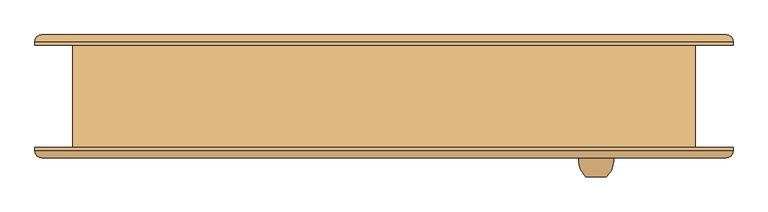
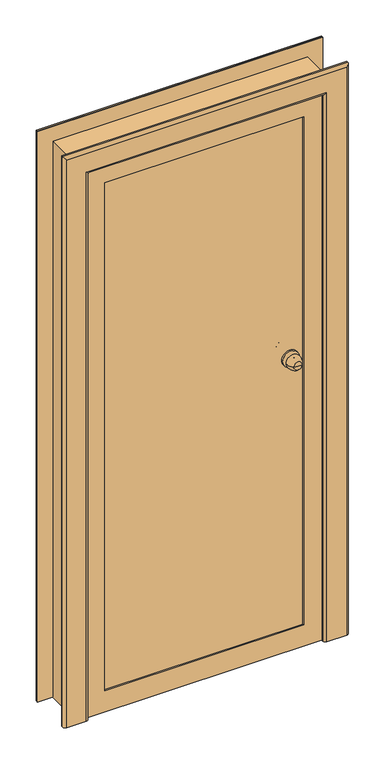
"""IFC4 building model written with IfcOpenShell, lengths in millimetres: door geometry, Наружная дверь 1-Навесная - Один проем наружу с порогом - 31173-2003 : ДСН КЛН  М1 УЗ 2100-910 ГОСТ 31173-2003."""

from ifc_helpers import new_model, si_unit, point, frame, origin, place, context, project, spatial, polyline, circle_curve, ellipse_curve, trimmed, outline, extrude, faceted_brep, source, transform, mapped, element, save
from ifc_brep_helpers import plane_surface, cylinder_surface, revolved_surface, advanced_brep


def door_a4fe4bf0(model_context):
    return source(origin(), model_context, "Body", "SolidModel", [
        advanced_brep(
        [(295.0, -118.0, 1100.0), (310.0, -118.0, 1100.0), (325.0, -118.0, 1100.0), (335.0, -88.0, 1100.0), (285.0, -88.0, 1100.0), (328.0, -88.0, 1100.0), (292.0, -88.0, 1100.0), (320.0, -80.0, 1100.0), (300.0, -80.0, 1100.0), (320.0, -74.0, 1100.0), (300.0, -74.0, 1100.0), (340.0, -74.0, 1100.0), (280.0, -74.0, 1100.0), (340.0, -68.0, 1100.0), (280.0, -68.0, 1100.0)],
        [
            (0, 1),
            (1, 2),
            (2, 0, circle_curve(frame((310.0, -118.0, 1100.0), z_axis=(0.0, -1.0, 0.0), x_axis=(1.0, 0.0, 0.0)), 15.0)),
            (0, 2, circle_curve(frame((310.0, -118.0, 1100.0), z_axis=(0.0, -1.0, 0.0), x_axis=(1.0, 0.0, 0.0)), 15.0)),
            (2, 3, circle_curve(frame((300.3773735, -93.1257912, 1100.0), z_axis=(0.0, 0.0, 1.0), x_axis=(-1.0, 0.0, 0.0)), 35.0)),
            (3, 4, circle_curve(frame((310.0, -88.0, 1100.0), z_axis=(0.0, -1.0, 0.0), x_axis=(1.0, 0.0, 0.0)), 25.0)),
            (4, 0, circle_curve(frame((319.6226265, -93.1257912, 1100.0), z_axis=(0.0, 0.0, 1.0), x_axis=(1.0, 0.0, 0.0)), 35.0)),
            (4, 3, circle_curve(frame((310.0, -88.0, 1100.0), z_axis=(0.0, -1.0, 0.0), x_axis=(1.0, 0.0, 0.0)), 25.0)),
            (3, 5),
            (5, 6, circle_curve(frame((310.0, -88.0, 1100.0), z_axis=(0.0, -1.0, 0.0), x_axis=(1.0, 0.0, 0.0)), 18.0)),
            (6, 4),
            (6, 5, circle_curve(frame((310.0, -88.0, 1100.0), z_axis=(0.0, -1.0, 0.0), x_axis=(1.0, 0.0, 0.0)), 18.0)),
            (5, 7, circle_curve(frame((328.0, -80.0, 1100.0), z_axis=(0.0, 0.0, -1.0), x_axis=(-1.0, 0.0, 0.0)), 8.0)),
            (7, 8, circle_curve(frame((310.0, -80.0, 1100.0), z_axis=(0.0, -1.0, 0.0), x_axis=(1.0, 0.0, 0.0)), 10.0)),
            (8, 6, circle_curve(frame((292.0, -80.0, 1100.0), z_axis=(0.0, 0.0, -1.0), x_axis=(1.0, 0.0, 0.0)), 8.0)),
            (8, 7, circle_curve(frame((310.0, -80.0, 1100.0), z_axis=(0.0, -1.0, 0.0), x_axis=(1.0, 0.0, 0.0)), 10.0)),
            (7, 9),
            (9, 10, circle_curve(frame((310.0, -74.0, 1100.0), z_axis=(0.0, -1.0, 0.0), x_axis=(1.0, 0.0, 0.0)), 10.0)),
            (10, 8),
            (10, 9, circle_curve(frame((310.0, -74.0, 1100.0), z_axis=(0.0, -1.0, 0.0), x_axis=(1.0, 0.0, 0.0)), 10.0)),
            (11, 12, circle_curve(frame((310.0, -74.0, 1100.0), z_axis=(0.0, -1.0, 0.0), x_axis=(-1.0, 0.0, 0.0)), 30.0)),
            (12, 11, circle_curve(frame((310.0, -74.0, 1100.0), z_axis=(0.0, -1.0, 0.0), x_axis=(-1.0, 0.0, 0.0)), 30.0)),
            (13, 14, circle_curve(frame((310.0, -68.0, 1100.0), z_axis=(0.0, 1.0, 0.0), x_axis=(-1.0, 0.0, 0.0)), 30.0)),
            (14, 13, circle_curve(frame((310.0, -68.0, 1100.0), z_axis=(0.0, 1.0, 0.0), x_axis=(-1.0, 0.0, 0.0)), 30.0)),
            (12, 14),
            (13, 11),
        ],
        [
            plane_surface(frame((310.0, -118.0, 1100.0), z_axis=(0.0, -1.0, 0.0), x_axis=(1.0, 0.0, 0.0))),
            revolved_surface(trimmed(ellipse_curve(frame((300.3773735, -93.1257912, 1100.0), z_axis=(0.0, 0.0, 1.0), x_axis=(-1.0, 0.0, 0.0)), 35.0, 35.0), [point((325.0, -118.0, 1100.0))], [point((335.0, -88.0, 1100.0))], True, "CARTESIAN"), (310.0, -148.0, 1100.0), (0.0, 1.0, 0.0)),
            plane_surface(frame((310.0, -88.0, 1100.0), z_axis=(0.0, 1.0, 0.0), x_axis=(1.0, 0.0, 0.0))),
            revolved_surface(trimmed(ellipse_curve(frame((328.0, -80.0, 1100.0), z_axis=(0.0, 0.0, -1.0), x_axis=(-1.0, 0.0, 0.0)), 8.0, 8.0), [point((328.0, -88.0, 1100.0))], [point((320.0, -80.0, 1100.0))], True, "CARTESIAN"), (310.0, -148.0, 1100.0), (0.0, 1.0, 0.0)),
            cylinder_surface(frame((310.0, -148.0, 1100.0), z_axis=(0.0, 1.0, 0.0), x_axis=(1.0, 0.0, 0.0)), 10.0),
            plane_surface(frame((280.0, -74.0, 1100.0), z_axis=(0.0, -1.0, 0.0), x_axis=(0.0, 0.0, 1.0))),
            plane_surface(frame((280.0, -68.0, 1100.0), z_axis=(0.0, 1.0, 0.0), x_axis=(0.0, 0.0, -1.0))),
            cylinder_surface(frame((310.0, -68.0, 1100.0), z_axis=(0.0, -1.0, 0.0), x_axis=(-1.0, 0.0, 0.0)), 30.0),
        ],
        [
            (0, [[1, 2, 3]]),
            (0, [[-1, 4, -2]]),
            (1, [[5, 6, 7, -3]]),
            (1, [[-7, 8, -5, -4]]),
            (2, [[9, 10, 11, -6]]),
            (2, [[-11, 12, -9, -8]]),
            (3, [[13, 14, 15, -10]]),
            (3, [[-15, 16, -13, -12]]),
            (4, [[17, 18, 19, -14]]),
            (4, [[-19, 20, -17, -16]]),
            (5, [[21, 22], [-20, -18]]),
            (6, [[23, 24]]),
            (7, [[25, -23, 26, -22]]),
            (7, [[-26, -24, -25, -21]]),
        ],
    ),
        advanced_brep(
        [(325.0, 52.0, 1100.0), (310.0, 52.0, 1100.0), (295.0, 52.0, 1100.0), (285.0, 22.0, 1100.0), (335.0, 22.0, 1100.0), (292.0, 22.0, 1100.0), (328.0, 22.0, 1100.0), (300.0, 14.0, 1100.0), (320.0, 14.0, 1100.0), (300.0, 8.0, 1100.0), (320.0, 8.0, 1100.0), (280.0, 8.0, 1100.0), (340.0, 8.0, 1100.0), (280.0, 2.0, 1100.0), (340.0, 2.0, 1100.0)],
        [
            (0, 1),
            (1, 2),
            (2, 0, circle_curve(frame((310.0, 52.0, 1100.0), z_axis=(0.0, 1.0, 0.0), x_axis=(-1.0, 0.0, 0.0)), 15.0)),
            (0, 2, circle_curve(frame((310.0, 52.0, 1100.0), z_axis=(0.0, 1.0, 0.0), x_axis=(-1.0, 0.0, 0.0)), 15.0)),
            (2, 3, circle_curve(frame((319.6226265, 27.1257912, 1100.0), z_axis=(0.0, 0.0, 1.0), x_axis=(1.0, 0.0, 0.0)), 35.0)),
            (3, 4, circle_curve(frame((310.0, 22.0, 1100.0), z_axis=(0.0, 1.0, 0.0), x_axis=(-1.0, 0.0, 0.0)), 25.0)),
            (4, 0, circle_curve(frame((300.3773735, 27.1257912, 1100.0), z_axis=(0.0, 0.0, 1.0), x_axis=(-1.0, 0.0, 0.0)), 35.0)),
            (4, 3, circle_curve(frame((310.0, 22.0, 1100.0), z_axis=(0.0, 1.0, 0.0), x_axis=(-1.0, 0.0, 0.0)), 25.0)),
            (3, 5),
            (5, 6, circle_curve(frame((310.0, 22.0, 1100.0), z_axis=(0.0, 1.0, 0.0), x_axis=(-1.0, 0.0, 0.0)), 18.0)),
            (6, 4),
            (6, 5, circle_curve(frame((310.0, 22.0, 1100.0), z_axis=(0.0, 1.0, 0.0), x_axis=(-1.0, 0.0, 0.0)), 18.0)),
            (5, 7, circle_curve(frame((292.0, 14.0, 1100.0), z_axis=(0.0, 0.0, -1.0), x_axis=(1.0, 0.0, 0.0)), 8.0)),
            (7, 8, circle_curve(frame((310.0, 14.0, 1100.0), z_axis=(0.0, 1.0, 0.0), x_axis=(-1.0, 0.0, 0.0)), 10.0)),
            (8, 6, circle_curve(frame((328.0, 14.0, 1100.0), z_axis=(0.0, 0.0, -1.0), x_axis=(-1.0, 0.0, 0.0)), 8.0)),
            (8, 7, circle_curve(frame((310.0, 14.0, 1100.0), z_axis=(0.0, 1.0, 0.0), x_axis=(-1.0, 0.0, 0.0)), 10.0)),
            (7, 9),
            (9, 10, circle_curve(frame((310.0, 8.0, 1100.0), z_axis=(0.0, 1.0, 0.0), x_axis=(-1.0, 0.0, 0.0)), 10.0)),
            (10, 8),
            (10, 9, circle_curve(frame((310.0, 8.0, 1100.0), z_axis=(0.0, 1.0, 0.0), x_axis=(-1.0, 0.0, 0.0)), 10.0)),
            (11, 12, circle_curve(frame((310.0, 8.0, 1100.0), z_axis=(0.0, 1.0, 0.0), x_axis=(1.0, 0.0, 0.0)), 30.0)),
            (12, 11, circle_curve(frame((310.0, 8.0, 1100.0), z_axis=(0.0, 1.0, 0.0), x_axis=(1.0, 0.0, 0.0)), 30.0)),
            (13, 14, circle_curve(frame((310.0, 2.0, 1100.0), z_axis=(0.0, -1.0, 0.0), x_axis=(1.0, 0.0, 0.0)), 30.0)),
            (14, 13, circle_curve(frame((310.0, 2.0, 1100.0), z_axis=(0.0, -1.0, 0.0), x_axis=(1.0, 0.0, 0.0)), 30.0)),
            (12, 14),
            (13, 11),
        ],
        [
            plane_surface(frame((310.0, 52.0, 1100.0), z_axis=(0.0, 1.0, 0.0), x_axis=(-1.0, 0.0, 0.0))),
            revolved_surface(trimmed(ellipse_curve(frame((319.6226265, 27.1257912, 1100.0), z_axis=(0.0, 0.0, 1.0), x_axis=(1.0, 0.0, 0.0)), 35.0, 35.0), [point((295.0, 52.0, 1100.0))], [point((285.0, 22.0, 1100.0))], True, "CARTESIAN"), (310.0, 82.0, 1100.0), (0.0, -1.0, 0.0)),
            plane_surface(frame((310.0, 22.0, 1100.0), z_axis=(0.0, -1.0, 0.0), x_axis=(-1.0, 0.0, 0.0))),
            revolved_surface(trimmed(ellipse_curve(frame((292.0, 14.0, 1100.0), z_axis=(0.0, 0.0, -1.0), x_axis=(1.0, 0.0, 0.0)), 8.0, 8.0), [point((292.0, 22.0, 1100.0))], [point((300.0, 14.0, 1100.0))], True, "CARTESIAN"), (310.0, 82.0, 1100.0), (0.0, -1.0, 0.0)),
            cylinder_surface(frame((310.0, 82.0, 1100.0), z_axis=(0.0, -1.0, 0.0), x_axis=(-1.0, 0.0, 0.0)), 10.0),
            plane_surface(frame((340.0, 8.0, 1100.0), z_axis=(0.0, 1.0, 0.0), x_axis=(0.0, 0.0, 1.0))),
            plane_surface(frame((340.0, 2.0, 1100.0), z_axis=(0.0, -1.0, 0.0), x_axis=(0.0, 0.0, -1.0))),
            cylinder_surface(frame((310.0, 2.0, 1100.0), z_axis=(0.0, 1.0, 0.0), x_axis=(1.0, 0.0, 0.0)), 30.0),
        ],
        [
            (0, [[1, 2, 3]]),
            (0, [[-1, 4, -2]]),
            (1, [[5, 6, 7, -3]]),
            (1, [[-7, 8, -5, -4]]),
            (2, [[9, 10, 11, -6]]),
            (2, [[-11, 12, -9, -8]]),
            (3, [[13, 14, 15, -10]]),
            (3, [[-15, 16, -13, -12]]),
            (4, [[17, 18, 19, -14]]),
            (4, [[-19, 20, -17, -16]]),
            (5, [[21, 22], [-20, -18]]),
            (6, [[23, 24]]),
            (7, [[25, -23, 26, -22]]),
            (7, [[-26, -24, -25, -21]]),
        ],
    ),
        faceted_brep([(390.0, 2.0, 42.0), (390.0, -3.0, 42.0), (-390.0, -3.0, 42.0), (-390.0, 2.0, 42.0), (390.0, 2.0, 2035.0), (390.0, -3.0, 2035.0), (-390.0, -3.0, 2035.0), (370.0, -3.0, 2015.0), (370.0, -3.0, 62.0), (-370.0, -3.0, 62.0), (-370.0, -3.0, 2015.0), (-390.0, 2.0, 2035.0), (370.0, -68.0, 2015.0), (370.0, -68.0, 62.0), (-370.0, -68.0, 62.0), (-370.0, -68.0, 2015.0)], [[[0, 1, 2, 3]], [[4, 5, 1, 0]], [[5, 6, 2, 1], [7, 8, 9, 10]], [[2, 6, 11, 3]], [[11, 4, 0, 3]], [[7, 12, 13, 8]], [[9, 8, 13, 14]], [[15, 10, 9, 14]], [[12, 15, 14, 13]], [[4, 11, 6, 5]], [[7, 10, 15, 12]]]),
        extrude(outline(polyline([(0.0, 420.0), (0.0, 435.0), (2080.0, 435.0), (2080.0, -435.0), (0.0, -435.0), (0.0, -420.0), (2065.0, -420.0), (2065.0, 420.0), (0.0, 420.0)])), frame((0.0, -5.0, 0.0), z_axis=(0.0, 1.0, 0.0), x_axis=(0.0, 0.0, 1.0)), (0.0, 0.0, 1.0), 80.0),
        faceted_brep([(435.0, -5.0, 0.0), (435.0, -75.0, 0.0), (-435.0, -75.0, 0.0), (-435.0, -5.0, 0.0), (-435.0, -75.0, 2080.0), (-435.0, -5.0, 2080.0), (435.0, -75.0, 2080.0), (-355.0, -75.0, 2000.0), (355.0, -75.0, 2000.0), (355.0, -75.0, 80.0), (-355.0, -75.0, 80.0), (435.0, -5.0, 2080.0), (-375.0, -5.0, 60.0), (375.0, -5.0, 60.0), (375.0, -5.0, 2020.0), (-375.0, -5.0, 2020.0), (375.0, -70.0, 60.0), (-375.0, -70.0, 60.0), (-375.0, -70.0, 2020.0), (375.0, -70.0, 2020.0), (-355.0, -70.0, 80.0), (355.0, -70.0, 80.0), (355.0, -70.0, 2000.0), (-355.0, -70.0, 2000.0)], [[[0, 1, 2, 3]], [[3, 2, 4, 5]], [[2, 1, 6, 4], [7, 8, 9, 10]], [[5, 11, 0, 3], [12, 13, 14, 15]], [[16, 13, 12, 17]], [[17, 12, 15, 18]], [[18, 19, 16, 17], [20, 21, 22, 23]], [[9, 21, 20, 10]], [[10, 20, 23, 7]], [[11, 6, 1, 0]], [[19, 14, 13, 16]], [[8, 22, 21, 9]], [[5, 4, 6, 11]], [[18, 15, 14, 19]], [[7, 23, 22, 8]]]),
        advanced_brep(
        [(-510.0, -75.0, 0.0), (-420.0, -75.0, 0.0), (-420.0, -80.0, 0.0), (-430.0, -90.0, 0.0), (-500.0, -90.0, 0.0), (-510.0, -80.0, 0.0), (-510.0, -75.0, 2155.0), (510.0, -75.0, 2155.0), (510.0, -75.0, 0.0), (420.0, -75.0, 0.0), (420.0, -75.0, 2065.0), (-420.0, -75.0, 2065.0), (-420.0, -80.0, 2065.0), (-430.0, -90.0, 2075.0), (430.0, -90.0, 2075.0), (430.0, -90.0, 0.0), (500.0, -90.0, 0.0), (500.0, -90.0, 2145.0), (-500.0, -90.0, 2145.0), (-510.0, -80.0, 2155.0), (510.0, -80.0, 2155.0), (510.0, -80.0, 0.0), (420.0, -80.0, 0.0), (420.0, -80.0, 2065.0)],
        [
            (0, 1),
            (1, 2),
            (2, 3, circle_curve(frame((-430.0, -80.0, 0.0), z_axis=(0.0, 0.0, -1.0), x_axis=(-1.0, 0.0, 0.0)), 10.0)),
            (3, 4),
            (4, 5, circle_curve(frame((-500.0, -80.0, 0.0), z_axis=(0.0, 0.0, -1.0), x_axis=(-1.0, 0.0, 0.0)), 10.0)),
            (5, 0),
            (0, 6),
            (6, 7),
            (7, 8),
            (8, 9),
            (9, 10),
            (10, 11),
            (11, 1),
            (11, 12),
            (12, 2),
            (12, 13, ellipse_curve(frame((-430.0, -80.0, 2075.0), z_axis=(-0.7071067811865475, 0.0, -0.7071067811865475), x_axis=(0.7071067811865474, 0.0, -0.7071067811865476)), 14.1421356, 10.0)),
            (13, 3),
            (13, 14),
            (14, 15),
            (15, 16),
            (16, 17),
            (17, 18),
            (18, 4),
            (18, 19, ellipse_curve(frame((-500.0, -80.0, 2145.0), z_axis=(-0.7071067811865475, 0.0, -0.7071067811865475), x_axis=(0.7071067811865474, 0.0, -0.7071067811865476)), 14.1421356, 10.0)),
            (19, 5),
            (19, 6),
            (7, 20),
            (20, 21),
            (21, 8),
            (21, 16, circle_curve(frame((500.0, -80.0, 0.0), z_axis=(0.0, 0.0, -1.0), x_axis=(1.0, 0.0, 0.0)), 10.0)),
            (15, 22, circle_curve(frame((430.0, -80.0, 0.0), z_axis=(0.0, 0.0, -1.0), x_axis=(1.0, 0.0, 0.0)), 10.0)),
            (22, 9),
            (23, 10),
            (22, 23),
            (14, 23, ellipse_curve(frame((430.0, -80.0, 2075.0), z_axis=(0.7071067811865475, 0.0, -0.7071067811865475), x_axis=(0.7071067811865474, 0.0, 0.7071067811865476)), 14.1421356, 10.0)),
            (20, 17, ellipse_curve(frame((500.0, -80.0, 2145.0), z_axis=(0.7071067811865475, 0.0, -0.7071067811865475), x_axis=(0.7071067811865474, 0.0, 0.7071067811865476)), 14.1421356, 10.0)),
            (23, 12),
            (20, 19),
        ],
        [
            plane_surface(frame((-455.0, -75.0, 0.0), z_axis=(0.0, 0.0, -1.0), x_axis=(0.0, -1.0, 0.0))),
            plane_surface(frame((-510.0, -75.0, 0.0), z_axis=(0.0, 1.0, 0.0), x_axis=(0.0, 0.0, 1.0))),
            plane_surface(frame((-420.0, -75.0, 0.0), z_axis=(1.0, 0.0, 0.0), x_axis=(0.0, 0.0, 1.0))),
            cylinder_surface(frame((-430.0, -80.0, 0.0), z_axis=(0.0, 0.0, -1.0), x_axis=(-1.0, 0.0, 0.0)), 10.0),
            plane_surface(frame((-430.0, -90.0, 0.0), z_axis=(0.0, -1.0, 0.0), x_axis=(0.0, 0.0, 1.0))),
            cylinder_surface(frame((-500.0, -80.0, 0.0), z_axis=(0.0, 0.0, -1.0), x_axis=(-1.0, 0.0, 0.0)), 10.0),
            plane_surface(frame((-510.0, -80.0, 0.0), z_axis=(-1.0, 0.0, 0.0), x_axis=(0.0, 0.0, 1.0))),
            plane_surface(frame((510.0, -80.0, 2155.0), z_axis=(1.0, 0.0, 0.0), x_axis=(0.0, 0.0, -1.0))),
            plane_surface(frame((455.0, -75.0, 0.0), z_axis=(0.0, 0.0, -1.0), x_axis=(0.0, -1.0, 0.0))),
            plane_surface(frame((420.0, -75.0, 2065.0), z_axis=(-1.0, 0.0, 0.0), x_axis=(0.0, 0.0, -1.0))),
            cylinder_surface(frame((430.0, -80.0, 2100.0), z_axis=(0.0, 0.0, 1.0), x_axis=(1.0, 0.0, 0.0)), 10.0),
            cylinder_surface(frame((500.0, -80.0, 2100.0), z_axis=(0.0, 0.0, 1.0), x_axis=(1.0, 0.0, 0.0)), 10.0),
            plane_surface(frame((-420.0, -75.0, 2065.0), z_axis=(0.0, 0.0, -1.0), x_axis=(1.0, 0.0, 0.0))),
            cylinder_surface(frame((-455.0, -80.0, 2075.0), z_axis=(-1.0, 0.0, 0.0), x_axis=(0.0, 0.0, 1.0)), 10.0),
            cylinder_surface(frame((-455.0, -80.0, 2145.0), z_axis=(-1.0, 0.0, 0.0), x_axis=(0.0, 0.0, 1.0)), 10.0),
            plane_surface(frame((-510.0, -80.0, 2155.0), z_axis=(0.0, 0.0, 1.0), x_axis=(1.0, 0.0, 0.0))),
        ],
        [
            (0, [[1, 2, 3, 4, 5, 6]]),
            (1, [[-1, 7, 8, 9, 10, 11, 12, 13]]),
            (2, [[-2, -13, 14, 15]]),
            (3, [[-3, -15, 16, 17]]),
            (4, [[-4, -17, 18, 19, 20, 21, 22, 23]]),
            (5, [[-5, -23, 24, 25]]),
            (6, [[-6, -25, 26, -7]]),
            (7, [[27, 28, 29, -9]]),
            (8, [[-29, 30, -20, 31, 32, -10]]),
            (9, [[33, -11, -32, 34]]),
            (10, [[35, -34, -31, -19]]),
            (11, [[36, -21, -30, -28]]),
            (12, [[-14, -12, -33, 37]]),
            (13, [[-16, -37, -35, -18]]),
            (14, [[-24, -22, -36, 38]]),
            (15, [[-26, -38, -27, -8]]),
        ],
    ),
        advanced_brep(
        [(510.0, 75.0, 0.0), (420.0, 75.0, 0.0), (420.0, 80.0, 0.0), (430.0, 90.0, 0.0), (500.0, 90.0, 0.0), (510.0, 80.0, 0.0), (510.0, 75.0, 2155.0), (-510.0, 75.0, 2155.0), (-510.0, 75.0, 0.0), (-420.0, 75.0, 0.0), (-420.0, 75.0, 2065.0), (420.0, 75.0, 2065.0), (420.0, 80.0, 2065.0), (430.0, 90.0, 2075.0), (-430.0, 90.0, 2075.0), (-430.0, 90.0, 0.0), (-500.0, 90.0, 0.0), (-500.0, 90.0, 2145.0), (500.0, 90.0, 2145.0), (510.0, 80.0, 2155.0), (-510.0, 80.0, 2155.0), (-510.0, 80.0, 0.0), (-420.0, 80.0, 0.0), (-420.0, 80.0, 2065.0)],
        [
            (0, 1),
            (1, 2),
            (2, 3, circle_curve(frame((430.0, 80.0, 0.0), z_axis=(0.0, 0.0, -1.0), x_axis=(1.0, 0.0, 0.0)), 10.0)),
            (3, 4),
            (4, 5, circle_curve(frame((500.0, 80.0, 0.0), z_axis=(0.0, 0.0, -1.0), x_axis=(1.0, 0.0, 0.0)), 10.0)),
            (5, 0),
            (0, 6),
            (6, 7),
            (7, 8),
            (8, 9),
            (9, 10),
            (10, 11),
            (11, 1),
            (11, 12),
            (12, 2),
            (12, 13, ellipse_curve(frame((430.0, 80.0, 2075.0), z_axis=(0.7071067811865475, 0.0, -0.7071067811865475), x_axis=(-0.7071067811865474, 0.0, -0.7071067811865476)), 14.1421356, 10.0)),
            (13, 3),
            (13, 14),
            (14, 15),
            (15, 16),
            (16, 17),
            (17, 18),
            (18, 4),
            (18, 19, ellipse_curve(frame((500.0, 80.0, 2145.0), z_axis=(0.7071067811865475, 0.0, -0.7071067811865475), x_axis=(-0.7071067811865474, 0.0, -0.7071067811865476)), 14.1421356, 10.0)),
            (19, 5),
            (19, 6),
            (7, 20),
            (20, 21),
            (21, 8),
            (21, 16, circle_curve(frame((-500.0, 80.0, 0.0), z_axis=(0.0, 0.0, -1.0), x_axis=(-1.0, 0.0, 0.0)), 10.0)),
            (15, 22, circle_curve(frame((-430.0, 80.0, 0.0), z_axis=(0.0, 0.0, -1.0), x_axis=(-1.0, 0.0, 0.0)), 10.0)),
            (22, 9),
            (23, 10),
            (22, 23),
            (14, 23, ellipse_curve(frame((-430.0, 80.0, 2075.0), z_axis=(-0.7071067811865475, 0.0, -0.7071067811865475), x_axis=(-0.7071067811865474, 0.0, 0.7071067811865476)), 14.1421356, 10.0)),
            (20, 17, ellipse_curve(frame((-500.0, 80.0, 2145.0), z_axis=(-0.7071067811865475, 0.0, -0.7071067811865475), x_axis=(-0.7071067811865474, 0.0, 0.7071067811865476)), 14.1421356, 10.0)),
            (23, 12),
            (20, 19),
        ],
        [
            plane_surface(frame((455.0, 75.0, 0.0), z_axis=(0.0, 0.0, -1.0), x_axis=(0.0, -1.0, 0.0))),
            plane_surface(frame((510.0, 75.0, 0.0), z_axis=(0.0, -1.0, 0.0), x_axis=(0.0, 0.0, 1.0))),
            plane_surface(frame((420.0, 75.0, 0.0), z_axis=(-1.0, 0.0, 0.0), x_axis=(0.0, 0.0, 1.0))),
            cylinder_surface(frame((430.0, 80.0, 0.0), z_axis=(0.0, 0.0, -1.0), x_axis=(1.0, 0.0, 0.0)), 10.0),
            plane_surface(frame((430.0, 90.0, 0.0), z_axis=(0.0, 1.0, 0.0), x_axis=(0.0, 0.0, 1.0))),
            cylinder_surface(frame((500.0, 80.0, 0.0), z_axis=(0.0, 0.0, -1.0), x_axis=(1.0, 0.0, 0.0)), 10.0),
            plane_surface(frame((510.0, 80.0, 0.0), z_axis=(1.0, 0.0, 0.0), x_axis=(0.0, 0.0, 1.0))),
            plane_surface(frame((-510.0, 80.0, 2155.0), z_axis=(-1.0, 0.0, 0.0), x_axis=(0.0, 0.0, -1.0))),
            plane_surface(frame((-455.0, 75.0, 0.0), z_axis=(0.0, 0.0, -1.0), x_axis=(0.0, -1.0, 0.0))),
            plane_surface(frame((-420.0, 75.0, 2065.0), z_axis=(1.0, 0.0, 0.0), x_axis=(0.0, 0.0, -1.0))),
            cylinder_surface(frame((-430.0, 80.0, 2100.0), z_axis=(0.0, 0.0, 1.0), x_axis=(-1.0, 0.0, 0.0)), 10.0),
            cylinder_surface(frame((-500.0, 80.0, 2100.0), z_axis=(0.0, 0.0, 1.0), x_axis=(-1.0, 0.0, 0.0)), 10.0),
            plane_surface(frame((420.0, 75.0, 2065.0), z_axis=(0.0, 0.0, -1.0), x_axis=(-1.0, 0.0, 0.0))),
            cylinder_surface(frame((455.0, 80.0, 2075.0), z_axis=(1.0, 0.0, 0.0), x_axis=(0.0, 0.0, 1.0)), 10.0),
            cylinder_surface(frame((455.0, 80.0, 2145.0), z_axis=(1.0, 0.0, 0.0), x_axis=(0.0, 0.0, 1.0)), 10.0),
            plane_surface(frame((510.0, 80.0, 2155.0), z_axis=(0.0, 0.0, 1.0), x_axis=(-1.0, 0.0, 0.0))),
        ],
        [
            (0, [[1, 2, 3, 4, 5, 6]]),
            (1, [[-1, 7, 8, 9, 10, 11, 12, 13]]),
            (2, [[-2, -13, 14, 15]]),
            (3, [[-3, -15, 16, 17]]),
            (4, [[-4, -17, 18, 19, 20, 21, 22, 23]]),
            (5, [[-5, -23, 24, 25]]),
            (6, [[-6, -25, 26, -7]]),
            (7, [[27, 28, 29, -9]]),
            (8, [[-29, 30, -20, 31, 32, -10]]),
            (9, [[33, -11, -32, 34]]),
            (10, [[35, -34, -31, -19]]),
            (11, [[36, -21, -30, -28]]),
            (12, [[-14, -12, -33, 37]]),
            (13, [[-16, -37, -35, -18]]),
            (14, [[-24, -22, -36, 38]]),
            (15, [[-26, -38, -27, -8]]),
        ],
    ),
        extrude(outline(polyline([(0.0, 435.0), (0.0, 455.0), (2100.0, 455.0), (2100.0, -455.0), (0.0, -455.0), (0.0, -435.0), (2080.0, -435.0), (2080.0, 435.0), (0.0, 435.0)])), frame((0.0, -75.0, 0.0), z_axis=(0.0, 1.0, 0.0), x_axis=(0.0, 0.0, 1.0)), (0.0, 0.0, 1.0), 150.0),
    ])


if __name__ == "__main__":
    model = new_model("IFC4")
    model_context = context("Model", 3, world=origin())
    ifc_project = project(units=[si_unit("LENGTHUNIT", "METRE", prefix="MILLI")], contexts=[model_context])
    site = spatial("IfcSite", under=ifc_project)
    building = spatial("IfcBuilding", under=site)
    placement = place(None, origin())
    door_shape = door_a4fe4bf0(model_context)
    element("IfcDoor", 1, ObjectType="Наружная дверь 1-Навесная - Один проем наружу с порогом - 31173-2003 : ДСН КЛН  М1 УЗ 2100-910 ГОСТ 31173-2003", at=placement, inside=building, context=model_context, shape_type="MappedRepresentation", body=[
        mapped(door_shape, transform((0.0, 0.0, 0.0), x_axis=(1.0, 0.0, 0.0), y_axis=(0.0, 1.0, 0.0), z_axis=(0.0, 0.0, 1.0))),
    ])
    save(model, "model.ifc")

# Revit data of these elements
# Type "Наружная дверь 1-Навесная - Один проем наружу с порогом - 31173-2003 : ДСН КЛН  М1 УЗ 2100-910 ГОСТ 31173-2003"
#   Type Mark = "156"
#   Description = "ДСН КЛН  М1 УЗ 2100-900 ГОСТ 31173-2003"
#   Проекционное соединение по ширине = 90 mm
#   Rough Width = 910 mm
#   Rough Height = 2100 mm
#   Угол проема [instance default] = 30°
#   Толщина_Тепл_Изоляции = 20 mm
#   Heat Transfer Coefficient (U) = 3.7021 W/(m²·K)
#   Height = 2080 mm
#   Width = 870 mm
#   Ширина каркаса = 60 mm
#   Толщина каркаса = 70 mm
#   Вставка двери [instance default] = 0 mm
#   Правая сторона = no
#   Левая сторона = yes
#   Function = 1
#   Обрезка = Сталь
#   Панель = Сталь
#   Тепловая изоляция = Тепловая изоляция
#   Кадр = Сталь
#   Дверная ручка = Металл
#   Visual Light Transmittance = 0
#   Solar Heat Gain Coefficient = 0
#   Construction Type Id = ""
#   Wall Closure = (empty or 0)
#   Analytic Construction = (empty or 0)
# Element 1 (IfcDoor, "Наружная дверь 1-Навесная - Один проем наружу с порогом - 31173-2003 : ДСН КЛН  М1 УЗ 2100-910 ГОСТ 31173-2003")
#   Materials on its faces: "Сталь", "Металл", "Тепловая изоляция"
# Materials
#   "Сталь": class "Металл", colour RGB 247 247 247, transparency 0
#   "Тепловая изоляция": class "Пластмасса", colour RGB 185 154 119, transparency 0, Cost = 0
#   "Металл": class "Металл", colour RGB 249 249 249, transparency 0
